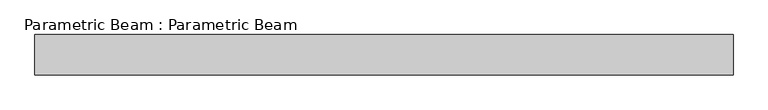
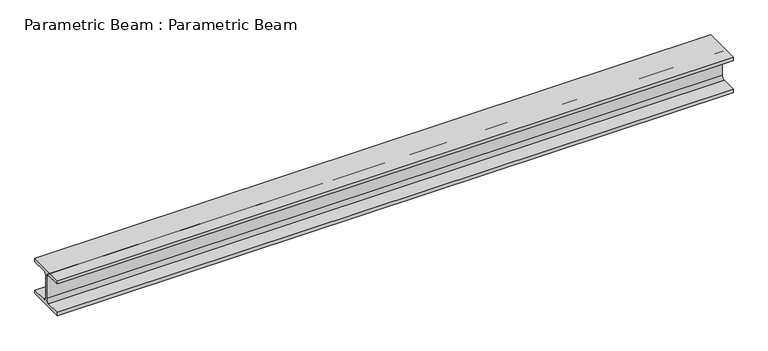
"""IFC4 building model written with IfcOpenShell, lengths in millimetres: beam geometry, Parametric Beam : Parametric Beam."""

from ifc_helpers import new_model, si_unit, point, frame, frame_2d, origin, place, context, project, spatial, polyline, circle_curve, trimmed, segment, composite_curve, outline, extrude, source, transform, mapped, element, save


def parametric_beam_parametric_beam_408cb472(model_context):
    return source(origin(), model_context, "Body", "SweptSolid", [
        extrude(outline(composite_curve([segment(polyline([(3.75, 72.0), (3.75, -72.0)]), True, "CONTINUOUS"), segment(trimmed(circle_curve(frame_2d((24.75, -72.0)), 21.0), [point((3.75, -72.0))], [point((24.75, -93.0))], True, "CARTESIAN"), True, "CONTINUOUS"), segment(polyline([(24.75, -93.0), (120.0, -93.0), (120.0, -115.0), (-120.0, -115.0), (-120.0, -93.0), (-24.75, -93.0)]), True, "CONTINUOUS"), segment(trimmed(circle_curve(frame_2d((-24.75, -72.0)), 21.0), [point((-24.75, -93.0))], [point((-3.75, -72.0))], True, "CARTESIAN"), True, "CONTINUOUS"), segment(polyline([(-3.75, -72.0), (-3.75, 72.0)]), True, "CONTINUOUS"), segment(trimmed(circle_curve(frame_2d((-24.75, 72.0)), 21.0), [point((-3.75, 72.0))], [point((-24.75, 93.0))], True, "CARTESIAN"), True, "CONTINUOUS"), segment(polyline([(-24.75, 93.0), (-120.0, 93.0), (-120.0, 115.0), (120.0, 115.0), (120.0, 93.0), (24.75, 93.0)]), True, "CONTINUOUS"), segment(trimmed(circle_curve(frame_2d((24.75, 72.0)), 21.0), [point((24.75, 93.0))], [point((3.75, 72.0))], True, "CARTESIAN"), True, "CONTINUOUS")], self_intersect=False)), frame((-2004.5455196, 0.0, 0.0), z_axis=(1.0, 0.0, 0.0), x_axis=(0.0, 1.0, 0.0)), (0.0, 0.0, 1.0), 4163.2589608),
    ])


if __name__ == "__main__":
    model = new_model("IFC4")
    model_context = context("Model", 3, world=origin())
    ifc_project = project(units=[si_unit("LENGTHUNIT", "METRE", prefix="MILLI")], contexts=[model_context])
    site = spatial("IfcSite", under=ifc_project)
    building = spatial("IfcBuilding", under=site)
    placement = place(None, origin())
    parametric_beam_parametric_beam_shape = parametric_beam_parametric_beam_408cb472(model_context)
    element("IfcBeam", 1, ObjectType="Parametric Beam : Parametric Beam", at=placement, inside=building, context=model_context, shape_type="MappedRepresentation", body=[
        mapped(parametric_beam_parametric_beam_shape, transform((0.0, 0.0, 0.0), x_axis=(1.0, 0.0, 0.0), y_axis=(0.0, 1.0, 0.0), z_axis=(0.0, 0.0, 1.0))),
    ])
    save(model, "model.ifc")

# Revit data of these elements
# Type "Parametric Beam : Parametric Beam"
#   MHP_PRO_Name [instance default] = "HEA"
#   r [instance default] = 0.021 m
#   h [instance default] = 0.3 m
#   b [instance default] = 0.24 m
#   Tw [instance default] = 0.0075 m
#   Tf [instance default] = 0.012 m
#   Length [instance default] = 3 m
#   Viktor_Change [instance default] = yes
# Element 1 (IfcBeam, "Parametric Beam : Parametric Beam")
#   MHP_PRO_Name = "HEA240"
#   h = 0.23 m
#   Tf = 0.022 m
#   Viktor_Change = no
